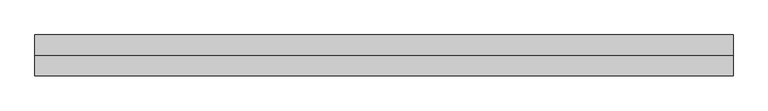
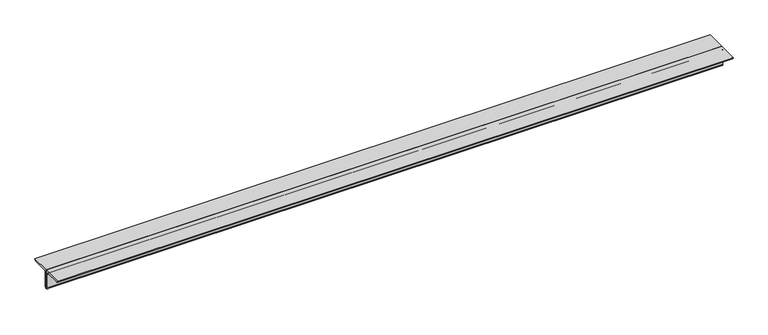
"""IFC4 building model written with IfcOpenShell, lengths in millimetres: beam geometry, 0123_Steel Framing_2Ls-KSD3502 : H_SB_AR_S04_2Ls-130x130x12_VBR1."""

from ifc_helpers import new_model, si_unit, point, frame, frame_2d, origin, place, context, project, spatial, polyline, circle_curve, trimmed, segment, composite_curve, outline, extrude, source, transform, mapped, element, save


def beam_1897c64a(model_context):
    return source(origin(), model_context, "Body", "SweptSolid", [
        extrude(outline(composite_curve([segment(polyline([(0.0, 36.4), (130.0, 36.4)]), True, "CONTINUOUS"), segment(trimmed(circle_curve(frame_2d((118.0, 36.4)), 12.0), [point((130.0, 36.4))], [point((118.0, 24.4))], False, "CARTESIAN"), True, "CONTINUOUS"), segment(polyline([(118.0, 24.4), (24.0, 24.4)]), True, "CONTINUOUS"), segment(trimmed(circle_curve(frame_2d((24.0, 12.4)), 12.0), [point((24.0, 24.4))], [point((12.0, 12.4))], True, "CARTESIAN"), True, "CONTINUOUS"), segment(polyline([(12.0, 12.4), (12.0, -81.6)]), True, "CONTINUOUS"), segment(trimmed(circle_curve(frame_2d((0.0, -81.6)), 12.0), [point((12.0, -81.6))], [point((0.0, -93.6))], False, "CARTESIAN"), True, "CONTINUOUS"), segment(polyline([(0.0, -93.6), (0.0, 36.4)]), True, "CONTINUOUS")], self_intersect=False)), frame((-2218.7564931, 0.0, 0.0), z_axis=(1.0, 0.0, 0.0), x_axis=(0.0, 1.0, 0.0)), (0.0, 0.0, 1.0), 4437.5129861),
        extrude(outline(composite_curve([segment(polyline([(0.0, 36.4), (0.0, -93.6)]), True, "CONTINUOUS"), segment(trimmed(circle_curve(frame_2d((0.0, -81.6)), 12.0), [point((0.0, -93.6))], [point((-12.0, -81.6))], False, "CARTESIAN"), True, "CONTINUOUS"), segment(polyline([(-12.0, -81.6), (-12.0, 12.4)]), True, "CONTINUOUS"), segment(trimmed(circle_curve(frame_2d((-24.0, 12.4)), 12.0), [point((-12.0, 12.4))], [point((-24.0, 24.4))], True, "CARTESIAN"), True, "CONTINUOUS"), segment(polyline([(-24.0, 24.4), (-118.0, 24.4)]), True, "CONTINUOUS"), segment(trimmed(circle_curve(frame_2d((-118.0, 36.4)), 12.0), [point((-118.0, 24.4))], [point((-130.0, 36.4))], False, "CARTESIAN"), True, "CONTINUOUS"), segment(polyline([(-130.0, 36.4), (0.0, 36.4)]), True, "CONTINUOUS")], self_intersect=False)), frame((-2218.7564931, 0.0, 0.0), z_axis=(1.0, 0.0, 0.0), x_axis=(0.0, 1.0, 0.0)), (0.0, 0.0, 1.0), 4437.5129861),
    ])


if __name__ == "__main__":
    model = new_model("IFC4")
    model_context = context("Model", 3, world=origin())
    ifc_project = project(units=[si_unit("LENGTHUNIT", "METRE", prefix="MILLI")], contexts=[model_context])
    site = spatial("IfcSite", under=ifc_project)
    building = spatial("IfcBuilding", under=site)
    placement = place(None, origin())
    beam_shape = beam_1897c64a(model_context)
    element("IfcBeam", 1, ObjectType="0123_Steel Framing_2Ls-KSD3502 : H_SB_AR_S04_2Ls-130x130x12_VBR1", at=placement, inside=building, context=model_context, shape_type="MappedRepresentation", body=[
        mapped(beam_shape, transform((0.0, 0.0, 0.0), x_axis=(1.0, 0.0, 0.0), y_axis=(0.0, 1.0, 0.0), z_axis=(0.0, 0.0, 1.0))),
    ])
    save(model, "model.ifc")

# Revit data of these elements
# Type "0123_Steel Framing_2Ls-KSD3502 : H_SB_AR_S04_2Ls-130x130x12_VBR1"
#   Type Mark = "VBR1"
#   Assembly Code = "B10"
#   Legs = "SLBB"
#   W = 8.97
#   Perimeter = 1.04 m²/m
#   Nominal Weight = 46.80 kgf/m
#   Length [instance default] = 1000 mm
#   Space = 0 mm
#   b = 130 mm
#   d = 130 mm
#   t = 12 mm
#   y = 36.4 mm
#   A = 0.005952 m²
#   Structural Material [instance default] = Steel ASTM A36
# Element 1 (IfcBeam, "0123_Steel Framing_2Ls-KSD3502 : H_SB_AR_S04_2Ls-130x130x12_VBR1")
#   Materials on its faces: "Steel ASTM A36"
# Materials
#   "Steel ASTM A36": class "Metal", colour RGB 199 199 199, transparency 0, Description = "Structural steel, ASTM A36 Grade B, mill finish", Cost = 0
